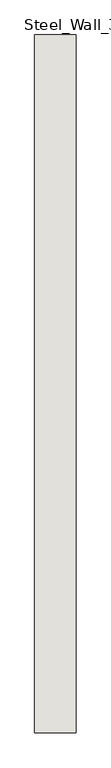
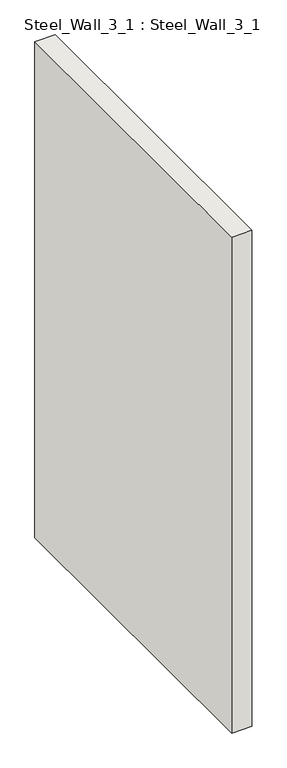
"""IFC4 building model written with IfcOpenShell, lengths in millimetres: wall geometry, Steel_Wall_3_1 : Steel_Wall_3_1."""

import ifcopenshell
import ifcopenshell.guid

model = None  # the IFC model being written
_history = None  # IfcOwnerHistory: only IFC2X3 demands one
_inside = {}  # id of a spatial element -> (the spatial element, [elements in it])
_under = {}  # id of a project, library or spatial element -> (it, [spatial elements below it])
_declared = {}  # id of a project -> (the project, [libraries it declares])
_typed = {}  # id of a type object -> (the type object, [elements of that type])
_made_of = {}  # id of a material, layer set ... -> (it, [elements and type objects made of it])


def new_model(schema):
    """Start an empty IFC model of exactly this schema.

    Asked for "IFC4X3", IfcOpenShell would pick the latest addendum, in which some entities
    have other attributes; the version numbers below select the first issue.
    IFC2X3 requires an IfcOwnerHistory on every rooted entity: one is made here for all.
    """
    global model, _history
    if schema == "IFC4X3":
        model = ifcopenshell.file(schema_version=(4, 3, 0, 0))
    else:
        model = ifcopenshell.file(schema=schema)
    _inside.clear()
    _under.clear()
    _declared.clear()
    _typed.clear()
    _made_of.clear()
    _history = None
    if model.schema == "IFC2X3":
        org = make("IfcOrganization", Name="unknown")
        user = make(
            "IfcPersonAndOrganization",
            ThePerson=make("IfcPerson", FamilyName="unknown"),
            TheOrganization=org,
        )
        app = make(
            "IfcApplication",
            ApplicationDeveloper=org,
            Version="unknown",
            ApplicationFullName="unknown",
            ApplicationIdentifier="unknown",
        )
        _history = make(
            "IfcOwnerHistory",
            OwningUser=user,
            OwningApplication=app,
            ChangeAction="ADDED",
            CreationDate=0,
        )
    return model


def make(cls, **values):
    """One entity of the class cls with the attributes given. An attribute that is None is left unset."""
    return model.create_entity(
        cls, **{name: value for name, value in values.items() if value is not None}
    )


def rooted(cls, **values):
    """An entity with a GlobalId (a new one), such as an element, a storey or a relation."""
    return make(cls, GlobalId=ifcopenshell.guid.new(), OwnerHistory=_history, **values)


def si_unit(unit_type, name, prefix=None):
    """IfcSIUnit, for example si_unit("LENGTHUNIT", "METRE", prefix="MILLI")."""
    return make("IfcSIUnit", UnitType=unit_type, Prefix=prefix, Name=name)


def assignment(units):
    """IfcUnitAssignment: the units of a project."""
    return None if units is None else make("IfcUnitAssignment", Units=units)


def point(xyz):
    """IfcCartesianPoint."""
    return None if xyz is None else make("IfcCartesianPoint", Coordinates=xyz)


def direction(xyz):
    """IfcDirection."""
    return None if xyz is None else make("IfcDirection", DirectionRatios=xyz)


def frame(location, z_axis=None, x_axis=None):
    """IfcAxis2Placement3D, a coordinate frame: its origin and axes. An axis left out is left unset."""
    return make(
        "IfcAxis2Placement3D",
        Location=point(location),
        Axis=direction(z_axis),
        RefDirection=direction(x_axis),
    )


def origin():
    """The frame at (0, 0, 0) with its axes left unset."""
    return frame((0.0, 0.0, 0.0))


def place(relative_to, where):
    """IfcLocalPlacement: puts the frame where relative to a parent placement (None: the world)."""
    return make(
        "IfcLocalPlacement", PlacementRelTo=relative_to, RelativePlacement=where
    )


def context(
    kind, dimensions, precision=None, world=None, true_north=None, identifier=None
):
    """IfcGeometricRepresentationContext, for example the 3D "Model" context."""
    return make(
        "IfcGeometricRepresentationContext",
        ContextIdentifier=identifier,
        ContextType=kind,
        CoordinateSpaceDimension=dimensions,
        Precision=precision,
        WorldCoordinateSystem=world,
        TrueNorth=true_north,
    )


def project(units=None, contexts=None):
    """IfcProject with its units and contexts."""
    return rooted(
        "IfcProject",
        Name="project",
        RepresentationContexts=contexts,
        UnitsInContext=assignment(units),
    )


def spatial(cls, under=None, at=None, **own):
    """A site, building, storey or space (cls), placed at a placement, below another one or the project."""
    s = rooted(cls, ObjectPlacement=at, **own)
    if under is not None:
        _under.setdefault(under.id(), (under, []))[1].append(s)
    return s


def polyline(points):
    """IfcPolyline through the points."""
    return make("IfcPolyline", Points=[point(p) for p in points])


def outline(outer, holes=None, kind="AREA"):
    """IfcArbitraryClosedProfileDef: a profile drawn as a closed curve; with holes, ...WithVoids."""
    if holes is None:
        return make("IfcArbitraryClosedProfileDef", ProfileType=kind, OuterCurve=outer)
    return make(
        "IfcArbitraryProfileDefWithVoids",
        ProfileType=kind,
        OuterCurve=outer,
        InnerCurves=holes,
    )


def extrude(swept, where, along, depth):
    """IfcExtrudedAreaSolid: the profile swept, set in the frame where, extruded along a direction by depth."""
    return make(
        "IfcExtrudedAreaSolid",
        SweptArea=swept,
        Position=where,
        ExtrudedDirection=direction(along),
        Depth=depth,
    )


def shape(context_of_items, identifier, shape_type, items):
    """IfcShapeRepresentation: the items that make up one representation, for example the "Body"."""
    return make(
        "IfcShapeRepresentation",
        ContextOfItems=context_of_items,
        RepresentationIdentifier=identifier,
        RepresentationType=shape_type,
        Items=items,
    )


def source(mapping_origin, context_of_items, identifier, shape_type, items):
    """IfcRepresentationMap: a shape defined once, which mapped items show again and again."""
    return make(
        "IfcRepresentationMap",
        MappingOrigin=mapping_origin,
        MappedRepresentation=shape(context_of_items, identifier, shape_type, items),
    )


def transform(
    local_origin,
    x_axis=None,
    y_axis=None,
    z_axis=None,
    scale=None,
    scale2=None,
    scale3=None,
    uniform=True,
):
    """IfcCartesianTransformationOperator3D, or its non-uniform kind. x_axis, y_axis, z_axis: its Axis1, 2, 3."""
    if uniform:
        return make(
            "IfcCartesianTransformationOperator3D",
            Axis1=direction(x_axis),
            Axis2=direction(y_axis),
            LocalOrigin=point(local_origin),
            Scale=scale,
            Axis3=direction(z_axis),
        )
    return make(
        "IfcCartesianTransformationOperator3DnonUniform",
        Axis1=direction(x_axis),
        Axis2=direction(y_axis),
        LocalOrigin=point(local_origin),
        Scale=scale,
        Axis3=direction(z_axis),
        Scale2=scale2,
        Scale3=scale3,
    )


def mapped(mapping_source, mapping_target):
    """IfcMappedItem: shows the shape of a source again, moved by a transform."""
    return make(
        "IfcMappedItem", MappingSource=mapping_source, MappingTarget=mapping_target
    )


def made_of(thing, what):
    """Note that an element or type object is made of a material, layer set ...; save() writes the relation."""
    if what is not None:
        _made_of.setdefault(what.id(), (what, []))[1].append(thing)
    return thing


def element(
    cls,
    number,
    at=None,
    inside=None,
    cuts=None,
    type_object=None,
    material=None,
    context=None,
    identifier="Body",
    shape_type=None,
    held_by="IfcProductDefinitionShape",
    body=None,
    shapes=None,
    **own,
):
    """One element of the class cls, such as IfcWall. Its Tag is "e" and its number.

    at: its placement. inside: the storey or other place that contains it. cuts: it is an
    opening in that element (IfcRelVoidsElement). A single representation is given by context,
    identifier, shape_type and body (its items); several are given by shapes. held_by: the class
    of the entity that holds the representations. save() writes the other relations.
    """
    e = rooted(cls, Tag="e%d" % number, ObjectPlacement=at, **own)
    if body is not None:
        shapes = [shape(context, identifier, shape_type, body)]
    if shapes is not None:
        e.Representation = make(held_by, Representations=shapes)
    if inside is not None:
        _inside.setdefault(inside.id(), (inside, []))[1].append(e)
    if cuts is not None:
        rooted(
            "IfcRelVoidsElement", RelatingBuildingElement=cuts, RelatedOpeningElement=e
        )
    if type_object is not None:
        _typed.setdefault(type_object.id(), (type_object, []))[1].append(e)
    return made_of(e, material)


def aggregate(whole, parts):
    """IfcRelAggregates: a whole, such as a stair, and the parts it consists of."""
    return rooted("IfcRelAggregates", RelatingObject=whole, RelatedObjects=parts)


def save(model, path):
    """Write the relations noted so far, then the file.

    IfcRelAggregates (storeys below a building ...), IfcRelContainedInSpatialStructure (elements
    in a storey), IfcRelDefinesByType, IfcRelAssociatesMaterial and IfcRelDeclares: one each for
    every whole, place, type object, material and project.
    """
    for whole, parts in _under.values():
        aggregate(whole, parts)
    for where, things in _inside.values():
        rooted(
            "IfcRelContainedInSpatialStructure",
            RelatedElements=things,
            RelatingStructure=where,
        )
    for kind, things in _typed.values():
        rooted("IfcRelDefinesByType", RelatedObjects=things, RelatingType=kind)
    for what, things in _made_of.values():
        rooted("IfcRelAssociatesMaterial", RelatedObjects=things, RelatingMaterial=what)
    for by, libraries in _declared.values():
        rooted("IfcRelDeclares", RelatingContext=by, RelatedDefinitions=libraries)
    model.write(path)


def steel_wall_3_1_steel_wall_3_1_bd8174d4(model_context):
    return source(origin(), model_context, "Body", "SweptSolid", [
        extrude(outline(polyline([(215.0, 9595.0), (215.0, 7905.0), (115.0, 7905.0), (115.0, 9595.0), (215.0, 9595.0)])), frame((0.0, 0.0, 250.0), z_axis=(0.0, 0.0, 1.0), x_axis=(1.0, 0.0, 0.0)), (0.0, 0.0, 1.0), 2600.0),
    ])


if __name__ == "__main__":
    model = new_model("IFC4")
    model_context = context("Model", 3, world=origin())
    ifc_project = project(units=[si_unit("LENGTHUNIT", "METRE", prefix="MILLI")], contexts=[model_context])
    site = spatial("IfcSite", under=ifc_project)
    building = spatial("IfcBuilding", under=site)
    placement = place(None, origin())
    steel_wall_3_1_steel_wall_3_1_shape = steel_wall_3_1_steel_wall_3_1_bd8174d4(model_context)
    element("IfcWall", 1, ObjectType="Steel_Wall_3_1 : Steel_Wall_3_1", at=placement, inside=building, context=model_context, shape_type="MappedRepresentation", body=[
        mapped(steel_wall_3_1_steel_wall_3_1_shape, transform((0.0, 0.0, 0.0), x_axis=(1.0, 0.0, 0.0), y_axis=(0.0, 1.0, 0.0), z_axis=(0.0, 0.0, 1.0))),
    ])
    save(model, "model.ifc")

# Revit data of these elements
# Type "Steel_Wall_3_1 : Steel_Wall_3_1"
#   NameOverride = "Steel_Wall_3_1"
# Element 1 (IfcWall, "Steel_Wall_3_1 : Steel_Wall_3_1")
#   Materials on its faces: "IfcSurfaceStyle #33"
# Materials
#   "IfcSurfaceStyle #33": class "Unassigned", colour RGB 214 214 214, transparency 0
